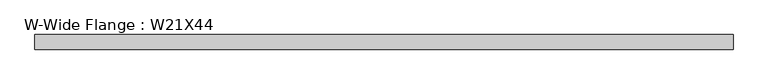
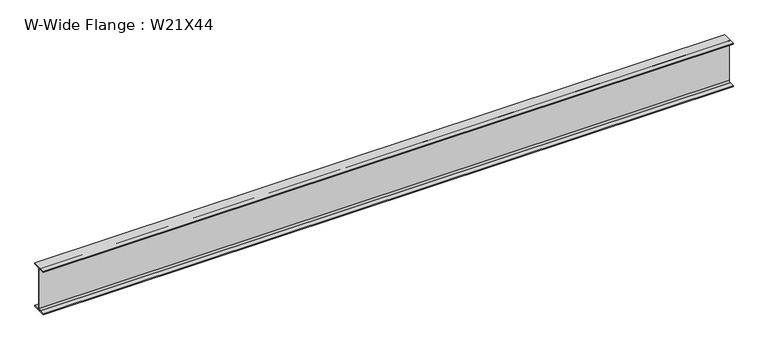
"""IFC4 building model written with IfcOpenShell, lengths in millimetres: beam geometry, W-Wide Flange : W21X44."""

from ifc_helpers import new_model, si_unit, point, frame, frame_2d, origin, place, context, project, spatial, polyline, circle_curve, trimmed, segment, composite_curve, outline, extrude, source, transform, mapped, element, save


def w_wide_flange_w21x44_6d4e9764(model_context):
    return source(origin(), model_context, "Body", "SweptSolid", [
        extrude(outline(composite_curve([segment(polyline([(82.55, -251.46), (82.55, -262.89), (-82.55, -262.89), (-82.55, -251.46), (-21.59, -251.46)]), True, "CONTINUOUS"), segment(trimmed(circle_curve(frame_2d((-21.59, -234.315)), 17.145), [point((-21.59, -251.46))], [point((-4.445, -234.315))], True, "CARTESIAN"), True, "CONTINUOUS"), segment(polyline([(-4.445, -234.315), (-4.445, 234.315)]), True, "CONTINUOUS"), segment(trimmed(circle_curve(frame_2d((-21.59, 234.315)), 17.145), [point((-4.445, 234.315))], [point((-21.59, 251.46))], True, "CARTESIAN"), True, "CONTINUOUS"), segment(polyline([(-21.59, 251.46), (-82.55, 251.46), (-82.55, 262.89), (82.55, 262.89), (82.55, 251.46), (21.59, 251.46)]), True, "CONTINUOUS"), segment(trimmed(circle_curve(frame_2d((21.59, 234.315)), 17.145), [point((21.59, 251.46))], [point((4.445, 234.315))], True, "CARTESIAN"), True, "CONTINUOUS"), segment(polyline([(4.445, 234.315), (4.445, -234.315)]), True, "CONTINUOUS"), segment(trimmed(circle_curve(frame_2d((21.59, -234.315)), 17.145), [point((4.445, -234.315))], [point((21.59, -251.46))], True, "CARTESIAN"), True, "CONTINUOUS"), segment(polyline([(21.59, -251.46), (82.55, -251.46)]), True, "CONTINUOUS")], self_intersect=False)), frame((-3910.3386404, 0.0, 0.0), z_axis=(1.0, 0.0, 0.0), x_axis=(0.0, 1.0, 0.0)), (0.0, 0.0, 1.0), 7881.257187),
    ])


if __name__ == "__main__":
    model = new_model("IFC4")
    model_context = context("Model", 3, world=origin())
    ifc_project = project(units=[si_unit("LENGTHUNIT", "METRE", prefix="MILLI")], contexts=[model_context])
    site = spatial("IfcSite", under=ifc_project)
    building = spatial("IfcBuilding", under=site)
    placement = place(None, origin())
    w_wide_flange_w21x44_shape = w_wide_flange_w21x44_6d4e9764(model_context)
    element("IfcBeam", 1, ObjectType="W-Wide Flange : W21X44", at=placement, inside=building, context=model_context, shape_type="MappedRepresentation", body=[
        mapped(w_wide_flange_w21x44_shape, transform((0.0, 0.0, 0.0), x_axis=(1.0, 0.0, 0.0), y_axis=(0.0, 1.0, 0.0), z_axis=(0.0, 0.0, 1.0))),
    ])
    save(model, "model.ifc")

# Revit data of these elements
# Type "W-Wide Flange : W21X44"
#   Assembly Code = "B10"
#   W = 44
#   Length [instance default] = 1524 mm
#   bf = 165.1 mm
#   d = 525.78 mm
#   k = 28.575 mm
#   k2 = 17.145 mm
#   tf = 11.43 mm
#   tw = 8.89 mm
#   A = 0.00838708 m²
#   Structural Material [instance default] = Steel ASTM A992
# Element 1 (IfcBeam, "W-Wide Flange : W21X44")
#   Structural Material = Aluminum, Anodized Red
#   Materials on its faces: "Aluminum, Anodized Red"
# Materials
#   "Steel ASTM A992": class "Metal", colour RGB 128 0 0, transparency 0, Description = "Structural steel 50ksi", Cost = 0
#   "Aluminum, Anodized Red": class "Metal", colour RGB 120 120 120, transparency 0, Description = "Anodized aluminum, red", Cost = 0
